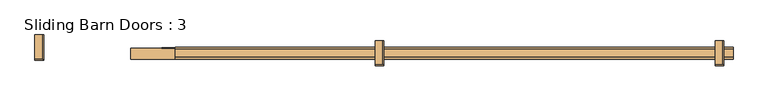
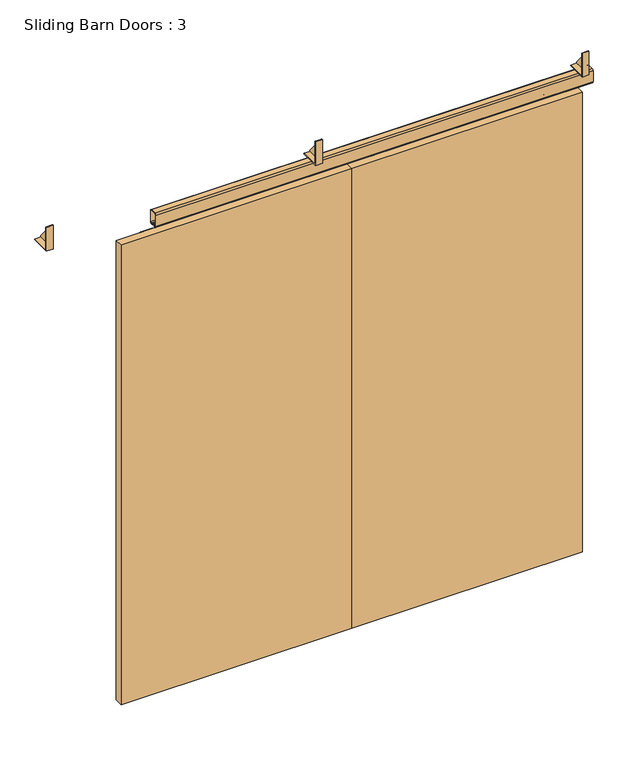
"""IFC4 building model written with IfcOpenShell, lengths in millimetres: door geometry, Sliding Barn Doors : 3."""

from ifc_helpers import new_model, si_unit, point, frame, frame_2d, origin, place, context, project, spatial, polyline, circle_curve, trimmed, segment, composite_curve, outline, extrude, source, transform, mapped, element, save


def sliding_barn_doors_3_b214497e(model_context):
    return source(origin(), model_context, "Body", "SweptSolid", [
        extrude(outline(polyline([(158.75, 2152.65), (158.75, 2146.3), (79.375, 2146.3), (79.375, 2247.773), (158.75, 2152.65)])), frame((-1330.3746094, 0.0, 0.0), z_axis=(1.0, 0.0, 0.0), x_axis=(0.0, 1.0, 0.0)), (0.0, 0.0, 1.0), 3.175),
        extrude(outline(polyline([(76.2, 2143.125), (76.2, 2247.773), (79.375, 2247.773), (79.375, 2146.3), (158.75, 2146.3), (158.75, 2143.125), (76.2, 2143.125)])), frame((-1355.6753906, 0.0, 0.0), z_axis=(1.0, 0.0, 0.0), x_axis=(0.0, 1.0, 0.0)), (0.0, 0.0, 1.0), 28.4757812),
        extrude(outline(polyline([(139.7, 2152.65), (139.7, 2146.3), (60.325, 2146.3), (60.325, 2247.773), (139.7, 2152.65)])), frame((-215.1558594, 0.0, 0.0), z_axis=(1.0, 0.0, 0.0), x_axis=(0.0, 1.0, 0.0)), (0.0, 0.0, 1.0), 3.175),
        extrude(outline(polyline([(57.15, 2143.125), (57.15, 2247.773), (60.325, 2247.773), (60.325, 2146.3), (139.7, 2146.3), (139.7, 2143.125), (57.15, 2143.125)])), frame((-240.4566406, 0.0, 0.0), z_axis=(1.0, 0.0, 0.0), x_axis=(0.0, 1.0, 0.0)), (0.0, 0.0, 1.0), 28.4757812),
        extrude(outline(polyline([(139.7, 2152.65), (139.7, 2146.3), (60.325, 2146.3), (60.325, 2247.773), (139.7, 2152.65)])), frame((900.0628906, 0.0, 0.0), z_axis=(1.0, 0.0, 0.0), x_axis=(0.0, 1.0, 0.0)), (0.0, 0.0, 1.0), 3.175),
        extrude(outline(polyline([(57.15, 2143.125), (57.15, 2247.773), (60.325, 2247.773), (60.325, 2146.3), (139.7, 2146.3), (139.7, 2143.125), (57.15, 2143.125)])), frame((874.7621094, 0.0, 0.0), z_axis=(1.0, 0.0, 0.0), x_axis=(0.0, 1.0, 0.0)), (0.0, 0.0, 1.0), 28.4757812),
        extrude(outline(polyline([(-940.054, 117.475), (-888.746, 117.475), (-888.746, 114.3), (-940.054, 114.3), (-940.054, 117.475)])), frame((0.0, 0.0, 1889.252), z_axis=(0.0, 0.0, 1.0), x_axis=(1.0, 0.0, 0.0)), (0.0, 0.0, 1.0), 168.148),
        extrude(outline(polyline([(-228.854, 117.475), (-177.546, 117.475), (-177.546, 114.3), (-228.854, 114.3), (-228.854, 117.475)])), frame((0.0, 0.0, 1889.252), z_axis=(0.0, 0.0, 1.0), x_axis=(1.0, 0.0, 0.0)), (0.0, 0.0, 1.0), 168.148),
        extrude(outline(polyline([(25.146, 117.475), (76.454, 117.475), (76.454, 114.3), (25.146, 114.3), (25.146, 117.475)])), frame((0.0, 0.0, 1889.252), z_axis=(0.0, 0.0, 1.0), x_axis=(1.0, 0.0, 0.0)), (0.0, 0.0, 1.0), 168.148),
        extrude(outline(polyline([(736.346, 117.475), (787.654, 117.475), (787.654, 114.3), (736.346, 114.3), (736.346, 117.475)])), frame((0.0, 0.0, 1889.252), z_axis=(0.0, 0.0, 1.0), x_axis=(1.0, 0.0, 0.0)), (0.0, 0.0, 1.0), 168.148),
        extrude(outline(polyline([(-1041.4, 114.3), (-76.2, 114.3), (-76.2, 79.375), (-1041.4, 79.375), (-1041.4, 114.3)])), frame((0.0, 0.0, 25.4), z_axis=(0.0, 0.0, 1.0), x_axis=(1.0, 0.0, 0.0)), (0.0, 0.0, 1.0), 2032.0),
        extrude(outline(polyline([(-76.2, 114.3), (889.0, 114.3), (889.0, 79.375), (-76.2, 79.375), (-76.2, 114.3)])), frame((0.0, 0.0, 25.4), z_axis=(0.0, 0.0, 1.0), x_axis=(1.0, 0.0, 0.0)), (0.0, 0.0, 1.0), 2032.0),
        extrude(outline(composite_curve([segment(polyline([(85.725, 2143.125), (111.252, 2143.125)]), True, "CONTINUOUS"), segment(trimmed(circle_curve(frame_2d((111.252, 2136.775)), 6.35), [point((111.252, 2143.125))], [point((117.602, 2136.775))], False, "CARTESIAN"), True, "CONTINUOUS"), segment(polyline([(117.602, 2136.775), (117.602, 2088.515)]), True, "CONTINUOUS"), segment(trimmed(circle_curve(frame_2d((111.252, 2088.515)), 6.35), [point((117.602, 2088.515))], [point((111.252, 2082.165))], False, "CARTESIAN"), True, "CONTINUOUS"), segment(polyline([(111.252, 2082.165), (105.8433147, 2082.165)]), True, "CONTINUOUS"), segment(trimmed(circle_curve(frame_2d((105.8433147, 2083.7525)), 1.5875), [point((105.8433147, 2082.165))], [point((104.2849816, 2083.4495907))], False, "CARTESIAN"), True, "CONTINUOUS"), segment(polyline([(104.2849816, 2083.4495907), (102.8594659, 2090.7832331), (104.3756029, 2090.7832331), (105.7615251, 2083.6532812), (111.252, 2083.6532812)]), True, "CONTINUOUS"), segment(trimmed(circle_curve(frame_2d((111.252, 2088.515)), 4.8617187), [point((111.252, 2083.6532812))], [point((116.1137188, 2088.515))], True, "CARTESIAN"), True, "CONTINUOUS"), segment(polyline([(116.1137188, 2088.515), (116.1137188, 2136.775)]), True, "CONTINUOUS"), segment(trimmed(circle_curve(frame_2d((111.252, 2136.775)), 4.8617187), [point((116.1137188, 2136.775))], [point((111.252, 2141.6367187))], True, "CARTESIAN"), True, "CONTINUOUS"), segment(polyline([(111.252, 2141.6367187), (85.725, 2141.6367187)]), True, "CONTINUOUS"), segment(trimmed(circle_curve(frame_2d((85.725, 2136.775)), 4.8617187), [point((85.725, 2141.6367187))], [point((80.8632813, 2136.775))], True, "CARTESIAN"), True, "CONTINUOUS"), segment(polyline([(80.8632813, 2136.775), (80.8632813, 2088.515)]), True, "CONTINUOUS"), segment(trimmed(circle_curve(frame_2d((85.725, 2088.515)), 4.8617187), [point((80.8632813, 2088.515))], [point((85.725, 2083.6532812))], True, "CARTESIAN"), True, "CONTINUOUS"), segment(polyline([(85.725, 2083.6532812), (91.2154749, 2083.6532812), (92.6013971, 2090.7832331), (94.1175341, 2090.7832331), (92.6920184, 2083.4495907)]), True, "CONTINUOUS"), segment(trimmed(circle_curve(frame_2d((91.1336853, 2083.7525)), 1.5875), [point((92.6920184, 2083.4495907))], [point((91.1336853, 2082.165))], False, "CARTESIAN"), True, "CONTINUOUS"), segment(polyline([(91.1336853, 2082.165), (85.725, 2082.165)]), True, "CONTINUOUS"), segment(trimmed(circle_curve(frame_2d((85.725, 2088.515)), 6.35), [point((85.725, 2082.165))], [point((79.375, 2088.515))], False, "CARTESIAN"), True, "CONTINUOUS"), segment(polyline([(79.375, 2088.515), (79.375, 2136.775)]), True, "CONTINUOUS"), segment(trimmed(circle_curve(frame_2d((85.725, 2136.775)), 6.35), [point((79.375, 2136.775))], [point((85.725, 2143.125))], False, "CARTESIAN"), True, "CONTINUOUS")], self_intersect=False)), frame((-895.35, 0.0, 0.0), z_axis=(1.0, 0.0, 0.0), x_axis=(0.0, 1.0, 0.0)), (0.0, 0.0, 1.0), 1828.8),
    ])


if __name__ == "__main__":
    model = new_model("IFC4")
    model_context = context("Model", 3, world=origin())
    ifc_project = project(units=[si_unit("LENGTHUNIT", "METRE", prefix="MILLI")], contexts=[model_context])
    site = spatial("IfcSite", under=ifc_project)
    building = spatial("IfcBuilding", under=site)
    placement = place(None, origin())
    sliding_barn_doors_3_shape = sliding_barn_doors_3_b214497e(model_context)
    element("IfcDoor", 1, ObjectType="Sliding Barn Doors : 3", at=placement, inside=building, context=model_context, shape_type="MappedRepresentation", body=[
        mapped(sliding_barn_doors_3_shape, transform((0.0, 0.0, 0.0), x_axis=(1.0, 0.0, 0.0), y_axis=(0.0, 1.0, 0.0), z_axis=(0.0, 0.0, 1.0))),
    ])
    save(model, "model.ifc")

# Revit data of these elements
# Type "Sliding Barn Doors : 3"
#   Type Mark = "43"
#   Analytic Construction = "<None>"
#   rail_overlap_left = 0' - 3 3/4"
#   rail_length = 6' - 0"
#   overlap_left = 0' - 2"
#   overlap = 0' - 0"
#   bracket_right = 1' - 7 13/16"
#   bracket_left = 0' - 2"
#   Thickness = 0' - 1 3/8"
#   Panel Width = 3' - 2"
#   Panel Height = 6' - 8"
#   Gap 2 = 0' - 0 1/2"
#   Gap 1 = 0' - 0 7/8"
#   Frame Projection Ext. = 0' - 1"
#   Frame Projection Int. = 0' - 1"
#   Frame Width = 0' - 3"
#   Height = 6' - 5 3/8"
#   Width = 5' - 6"
#   Bracket_offset = 0' - 5"
#   Door_4 = no
#   Door_3 = no
#   Hardware Material = Metal - Aluminum
#   Door Material = Closet_1
#   Function = (empty or 0)
#   Wall Closure = (empty or 0)
# Element 1 (IfcDoor, "Sliding Barn Doors : 3")
#   Materials on its faces: "Metal - Aluminum", "Closet_1"
# Materials
#   "Metal - Aluminum": class "Metal", colour RGB 247 247 247, transparency 0
#   "Closet_1": class "Paint", colour RGB 58 62 47, transparency 0, Cost = 0
